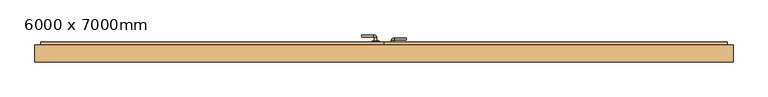
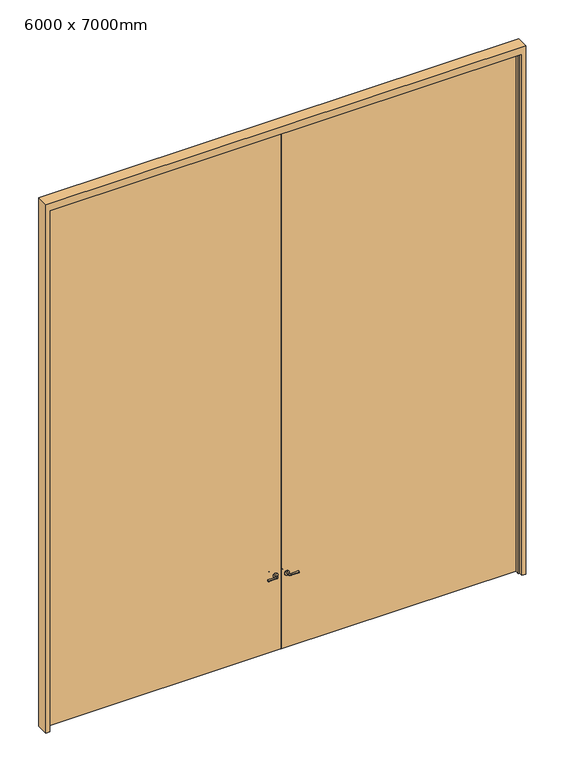
"""IFC4 building model written with IfcOpenShell, lengths in millimetres: door geometry, M_Puerta-De_paso-Doble-Paneles_planos : 6000 x 7000mm."""

from ifc_helpers import new_model, si_unit, point, frame, frame_2d, origin, origin_with_axes, place, context, project, spatial, polyline, circle_curve, ellipse_curve, trimmed, segment, composite_curve, outline, extrude, faceted_brep, source, transform, mapped, element, save
from ifc_brep_helpers import plane_surface, cylinder_surface, revolved_surface, advanced_brep


def door_6000_x_7000mm_428d85bf(model_context):
    return source(origin(), model_context, "Body", "SolidModel", [
        advanced_brep(
        [(-65.009375, 3.35, 1016.0), (-85.009375, 3.35, 1016.0), (-65.009375, -26.65, 1016.0), (-85.009375, -26.65, 1016.0), (-90.009375, -31.65, 1016.0), (-90.009375, -51.65, 1016.0), (-195.009375, -51.65, 1016.0), (-195.009375, -31.65, 1016.0)],
        [
            (0, 1, circle_curve(frame((-75.009375, 3.35, 1016.0), z_axis=(0.0, 1.0, 0.0), x_axis=(-1.0, 0.0, 0.0)), 10.0)),
            (1, 0, circle_curve(frame((-75.009375, 3.35, 1016.0), z_axis=(0.0, 1.0, 0.0), x_axis=(-1.0, 0.0, 0.0)), 10.0)),
            (0, 2),
            (2, 3, circle_curve(frame((-75.009375, -26.65, 1016.0), z_axis=(0.0, 1.0, 0.0), x_axis=(-1.0, 0.0, 0.0)), 10.0)),
            (3, 1),
            (3, 2, circle_curve(frame((-75.009375, -26.65, 1016.0), z_axis=(0.0, 1.0, 0.0), x_axis=(-1.0, 0.0, 0.0)), 10.0)),
            (4, 3, circle_curve(frame((-90.009375, -26.65, 1016.0), z_axis=(0.0, 0.0, 1.0), x_axis=(1.0, 0.0, 0.0)), 5.0)),
            (2, 5, circle_curve(frame((-90.009375, -26.65, 1016.0), z_axis=(0.0, 0.0, -1.0), x_axis=(1.0, 0.0, 0.0)), 25.0)),
            (5, 4, circle_curve(frame((-90.009375, -41.65, 1016.0), z_axis=(1.0, 0.0, 0.0), x_axis=(0.0, 1.0, 0.0)), 10.0)),
            (4, 5, circle_curve(frame((-90.009375, -41.65, 1016.0), z_axis=(1.0, 0.0, 0.0), x_axis=(0.0, 1.0, 0.0)), 10.0)),
            (6, 7, circle_curve(frame((-195.009375, -41.65, 1016.0), z_axis=(-1.0, 0.0, 0.0), x_axis=(0.0, 1.0, 0.0)), 10.0)),
            (7, 6, circle_curve(frame((-195.009375, -41.65, 1016.0), z_axis=(-1.0, 0.0, 0.0), x_axis=(0.0, 1.0, 0.0)), 10.0)),
            (5, 6),
            (7, 4),
        ],
        [
            plane_surface(frame((-75.009375, 3.35, 1016.0), z_axis=(0.0, 1.0, 0.0), x_axis=(0.0, 0.0, 1.0))),
            cylinder_surface(frame((-75.009375, 3.35, 1016.0), z_axis=(0.0, 1.0, 0.0), x_axis=(-1.0, 0.0, 0.0)), 10.0),
            revolved_surface(trimmed(ellipse_curve(frame((-75.009375, -26.65, 1016.0), z_axis=(0.0, 1.0, 0.0), x_axis=(-1.0, 0.0, 0.0)), 10.0, 10.0), [point((-65.009375, -26.65, 1016.0))], [point((-85.009375, -26.65, 1016.0))], True, "CARTESIAN"), (-90.009375, -26.65, 1016.0), (0.0, 0.0, -1.0)),
            revolved_surface(trimmed(ellipse_curve(frame((-75.009375, -26.65, 1016.0), z_axis=(0.0, 1.0, 0.0), x_axis=(-1.0, 0.0, 0.0)), 10.0, 10.0), [point((-85.009375, -26.65, 1016.0))], [point((-65.009375, -26.65, 1016.0))], True, "CARTESIAN"), (-90.009375, -26.65, 1016.0), (0.0, 0.0, -1.0)),
            plane_surface(frame((-195.009375, -41.65, 1016.0), z_axis=(-1.0, 0.0, 0.0), x_axis=(0.0, 0.0, 1.0))),
            cylinder_surface(frame((-90.009375, -41.65, 1016.0), z_axis=(1.0, 0.0, 0.0), x_axis=(0.0, 1.0, 0.0)), 10.0),
        ],
        [
            (0, [[1, 2]]),
            (1, [[-1, 3, 4, 5]]),
            (1, [[-2, -5, 6, -3]]),
            (2, [[7, -4, 8, 9]]),
            (3, [[-8, -6, -7, 10]]),
            (4, [[11, 12]]),
            (5, [[-9, 13, -12, 14]]),
            (5, [[-10, -14, -11, -13]]),
        ],
    ),
        extrude(outline(composite_curve([segment(trimmed(circle_curve(frame_2d((1016.0, -72.509375)), 30.0), [point((1016.0, -42.509375))], [point((1016.0, -102.509375))], False, "CARTESIAN"), True, "CONTINUOUS"), segment(trimmed(circle_curve(frame_2d((1016.0, -72.509375)), 30.0), [point((1016.0, -102.509375))], [point((1016.0, -42.509375))], False, "CARTESIAN"), True, "CONTINUOUS")], self_intersect=False)), frame((0.0, 3.35, 0.0), z_axis=(0.0, 1.0, 0.0), x_axis=(0.0, 0.0, 1.0)), (0.0, 0.0, 1.0), 8.0),
        advanced_brep(
        [(-65.009375, 90.95, 1000.0), (-85.009375, 90.95, 1000.0), (-85.009375, 120.95, 1000.0), (-65.009375, 120.95, 1000.0), (-90.009375, 125.95, 1000.0), (-90.009375, 145.95, 1000.0), (-195.009375, 145.95, 1000.0), (-195.009375, 125.95, 1000.0)],
        [
            (0, 1, circle_curve(frame((-75.009375, 90.95, 1000.0), z_axis=(0.0, -1.0, 0.0), x_axis=(-1.0, 0.0, 0.0)), 10.0)),
            (1, 0, circle_curve(frame((-75.009375, 90.95, 1000.0), z_axis=(0.0, -1.0, 0.0), x_axis=(-1.0, 0.0, 0.0)), 10.0)),
            (1, 2),
            (2, 3, circle_curve(frame((-75.009375, 120.95, 1000.0), z_axis=(0.0, -1.0, 0.0), x_axis=(-1.0, 0.0, 0.0)), 10.0)),
            (3, 0),
            (3, 2, circle_curve(frame((-75.009375, 120.95, 1000.0), z_axis=(0.0, -1.0, 0.0), x_axis=(-1.0, 0.0, 0.0)), 10.0)),
            (4, 5, circle_curve(frame((-90.009375, 135.95, 1000.0), z_axis=(1.0, 0.0, 0.0), x_axis=(0.0, -1.0, 0.0)), 10.0)),
            (5, 3, circle_curve(frame((-90.009375, 120.95, 1000.0), z_axis=(0.0, 0.0, -1.0), x_axis=(1.0, 0.0, 0.0)), 25.0)),
            (2, 4, circle_curve(frame((-90.009375, 120.95, 1000.0), z_axis=(0.0, 0.0, 1.0), x_axis=(1.0, 0.0, 0.0)), 5.0)),
            (5, 4, circle_curve(frame((-90.009375, 135.95, 1000.0), z_axis=(1.0, 0.0, 0.0), x_axis=(0.0, -1.0, 0.0)), 10.0)),
            (6, 7, circle_curve(frame((-195.009375, 135.95, 1000.0), z_axis=(-1.0, 0.0, 0.0), x_axis=(0.0, -1.0, 0.0)), 10.0)),
            (7, 6, circle_curve(frame((-195.009375, 135.95, 1000.0), z_axis=(-1.0, 0.0, 0.0), x_axis=(0.0, -1.0, 0.0)), 10.0)),
            (4, 7),
            (6, 5),
        ],
        [
            plane_surface(frame((-75.009375, 90.95, 1000.0), z_axis=(0.0, -1.0, 0.0), x_axis=(0.0, 0.0, 1.0))),
            cylinder_surface(frame((-75.009375, 90.95, 1000.0), z_axis=(0.0, -1.0, 0.0), x_axis=(-1.0, 0.0, 0.0)), 10.0),
            revolved_surface(trimmed(ellipse_curve(frame((-75.009375, 120.95, 1000.0), z_axis=(0.0, 1.0, 0.0), x_axis=(-1.0, 0.0, 0.0)), 10.0, 10.0), [point((-65.009375, 120.95, 1000.0))], [point((-85.009375, 120.95, 1000.0))], True, "CARTESIAN"), (-90.009375, 120.95, 1000.0), (0.0, 0.0, -1.0)),
            revolved_surface(trimmed(ellipse_curve(frame((-75.009375, 120.95, 1000.0), z_axis=(0.0, 1.0, 0.0), x_axis=(-1.0, 0.0, 0.0)), 10.0, 10.0), [point((-85.009375, 120.95, 1000.0))], [point((-65.009375, 120.95, 1000.0))], True, "CARTESIAN"), (-90.009375, 120.95, 1000.0), (0.0, 0.0, -1.0)),
            plane_surface(frame((-195.009375, 135.95, 1000.0), z_axis=(-1.0, 0.0, 0.0), x_axis=(0.0, 0.0, 1.0))),
            cylinder_surface(frame((-90.009375, 135.95, 1000.0), z_axis=(1.0, 0.0, 0.0), x_axis=(0.0, -1.0, 0.0)), 10.0),
        ],
        [
            (0, [[1, 2]]),
            (1, [[3, 4, 5, -2]]),
            (1, [[-5, 6, -3, -1]]),
            (2, [[7, 8, -4, 9]]),
            (3, [[10, -9, -6, -8]]),
            (4, [[11, 12]]),
            (5, [[13, -11, 14, -7]]),
            (5, [[-14, -12, -13, -10]]),
        ],
    ),
        extrude(outline(composite_curve([segment(trimmed(circle_curve(frame_2d((1000.0, -72.509375)), 30.0), [point((1000.0, -42.509375))], [point((1000.0, -102.509375))], False, "CARTESIAN"), True, "CONTINUOUS"), segment(trimmed(circle_curve(frame_2d((1000.0, -72.509375)), 30.0), [point((1000.0, -102.509375))], [point((1000.0, -42.509375))], False, "CARTESIAN"), True, "CONTINUOUS")], self_intersect=False)), frame((0.0, 82.95, 0.0), z_axis=(0.0, 1.0, 0.0), x_axis=(0.0, 0.0, 1.0)), (0.0, 0.0, 1.0), 8.0),
        advanced_brep(
        [(65.009375, 3.35, 1000.0), (85.009375, 3.35, 1000.0), (85.009375, -26.65, 1000.0), (65.009375, -26.65, 1000.0), (90.009375, -31.65, 1000.0), (90.009375, -51.65, 1000.0), (195.009375, -51.65, 1000.0), (195.009375, -31.65, 1000.0)],
        [
            (0, 1, circle_curve(frame((75.009375, 3.35, 1000.0), z_axis=(0.0, 1.0, 0.0), x_axis=(1.0, 0.0, 0.0)), 10.0)),
            (1, 0, circle_curve(frame((75.009375, 3.35, 1000.0), z_axis=(0.0, 1.0, 0.0), x_axis=(1.0, 0.0, 0.0)), 10.0)),
            (1, 2),
            (2, 3, circle_curve(frame((75.009375, -26.65, 1000.0), z_axis=(0.0, 1.0, 0.0), x_axis=(1.0, 0.0, 0.0)), 10.0)),
            (3, 0),
            (3, 2, circle_curve(frame((75.009375, -26.65, 1000.0), z_axis=(0.0, 1.0, 0.0), x_axis=(1.0, 0.0, 0.0)), 10.0)),
            (4, 5, circle_curve(frame((90.009375, -41.65, 1000.0), z_axis=(-1.0, 0.0, 0.0), x_axis=(0.0, 1.0, 0.0)), 10.0)),
            (5, 3, circle_curve(frame((90.009375, -26.65, 1000.0), z_axis=(0.0, 0.0, -1.0), x_axis=(-1.0, 0.0, 0.0)), 25.0)),
            (2, 4, circle_curve(frame((90.009375, -26.65, 1000.0), z_axis=(0.0, 0.0, 1.0), x_axis=(-1.0, 0.0, 0.0)), 5.0)),
            (5, 4, circle_curve(frame((90.009375, -41.65, 1000.0), z_axis=(-1.0, 0.0, 0.0), x_axis=(0.0, 1.0, 0.0)), 10.0)),
            (6, 7, circle_curve(frame((195.009375, -41.65, 1000.0), z_axis=(1.0, 0.0, 0.0), x_axis=(0.0, 1.0, 0.0)), 10.0)),
            (7, 6, circle_curve(frame((195.009375, -41.65, 1000.0), z_axis=(1.0, 0.0, 0.0), x_axis=(0.0, 1.0, 0.0)), 10.0)),
            (4, 7),
            (6, 5),
        ],
        [
            plane_surface(frame((75.009375, 3.35, 1000.0), z_axis=(0.0, 1.0, 0.0), x_axis=(0.0, 0.0, 1.0))),
            cylinder_surface(frame((75.009375, 3.35, 1000.0), z_axis=(0.0, 1.0, 0.0), x_axis=(1.0, 0.0, 0.0)), 10.0),
            revolved_surface(trimmed(ellipse_curve(frame((75.009375, -26.65, 1000.0), z_axis=(0.0, -1.0, 0.0), x_axis=(1.0, 0.0, 0.0)), 10.0, 10.0), [point((65.009375, -26.65, 1000.0))], [point((85.009375, -26.65, 1000.0))], True, "CARTESIAN"), (90.009375, -26.65, 1000.0), (0.0, 0.0, -1.0)),
            revolved_surface(trimmed(ellipse_curve(frame((75.009375, -26.65, 1000.0), z_axis=(0.0, -1.0, 0.0), x_axis=(1.0, 0.0, 0.0)), 10.0, 10.0), [point((85.009375, -26.65, 1000.0))], [point((65.009375, -26.65, 1000.0))], True, "CARTESIAN"), (90.009375, -26.65, 1000.0), (0.0, 0.0, -1.0)),
            plane_surface(frame((195.009375, -41.65, 1000.0), z_axis=(1.0, 0.0, 0.0), x_axis=(0.0, 0.0, 1.0))),
            cylinder_surface(frame((90.009375, -41.65, 1000.0), z_axis=(-1.0, 0.0, 0.0), x_axis=(0.0, 1.0, 0.0)), 10.0),
        ],
        [
            (0, [[1, 2]]),
            (1, [[3, 4, 5, -2]]),
            (1, [[-5, 6, -3, -1]]),
            (2, [[7, 8, -4, 9]]),
            (3, [[10, -9, -6, -8]]),
            (4, [[11, 12]]),
            (5, [[13, -11, 14, -7]]),
            (5, [[-14, -12, -13, -10]]),
        ],
    ),
        extrude(outline(composite_curve([segment(trimmed(circle_curve(frame_2d((1000.0, 72.509375)), 30.0), [point((1000.0, 42.509375))], [point((1000.0, 102.509375))], False, "CARTESIAN"), True, "CONTINUOUS"), segment(trimmed(circle_curve(frame_2d((1000.0, 72.509375)), 30.0), [point((1000.0, 102.509375))], [point((1000.0, 42.509375))], False, "CARTESIAN"), True, "CONTINUOUS")], self_intersect=False)), frame((0.0, 3.35, 0.0), z_axis=(0.0, 1.0, 0.0), x_axis=(0.0, 0.0, 1.0)), (0.0, 0.0, 1.0), 8.0),
        advanced_brep(
        [(65.009375, 64.35, 1000.0), (85.009375, 64.35, 1000.0), (65.009375, 94.35, 1000.0), (85.009375, 94.35, 1000.0), (90.009375, 99.35, 1000.0), (90.009375, 119.35, 1000.0), (195.009375, 119.35, 1000.0), (195.009375, 99.35, 1000.0)],
        [
            (0, 1, circle_curve(frame((75.009375, 64.35, 1000.0), z_axis=(0.0, -1.0, 0.0), x_axis=(1.0, 0.0, 0.0)), 10.0)),
            (1, 0, circle_curve(frame((75.009375, 64.35, 1000.0), z_axis=(0.0, -1.0, 0.0), x_axis=(1.0, 0.0, 0.0)), 10.0)),
            (0, 2),
            (2, 3, circle_curve(frame((75.009375, 94.35, 1000.0), z_axis=(0.0, -1.0, 0.0), x_axis=(1.0, 0.0, 0.0)), 10.0)),
            (3, 1),
            (3, 2, circle_curve(frame((75.009375, 94.35, 1000.0), z_axis=(0.0, -1.0, 0.0), x_axis=(1.0, 0.0, 0.0)), 10.0)),
            (4, 3, circle_curve(frame((90.009375, 94.35, 1000.0), z_axis=(0.0, 0.0, 1.0), x_axis=(-1.0, 0.0, 0.0)), 5.0)),
            (2, 5, circle_curve(frame((90.009375, 94.35, 1000.0), z_axis=(0.0, 0.0, -1.0), x_axis=(-1.0, 0.0, 0.0)), 25.0)),
            (5, 4, circle_curve(frame((90.009375, 109.35, 1000.0), z_axis=(-1.0, 0.0, 0.0), x_axis=(0.0, -1.0, 0.0)), 10.0)),
            (4, 5, circle_curve(frame((90.009375, 109.35, 1000.0), z_axis=(-1.0, 0.0, 0.0), x_axis=(0.0, -1.0, 0.0)), 10.0)),
            (6, 7, circle_curve(frame((195.009375, 109.35, 1000.0), z_axis=(1.0, 0.0, 0.0), x_axis=(0.0, -1.0, 0.0)), 10.0)),
            (7, 6, circle_curve(frame((195.009375, 109.35, 1000.0), z_axis=(1.0, 0.0, 0.0), x_axis=(0.0, -1.0, 0.0)), 10.0)),
            (5, 6),
            (7, 4),
        ],
        [
            plane_surface(frame((75.009375, 64.35, 1000.0), z_axis=(0.0, -1.0, 0.0), x_axis=(0.0, 0.0, 1.0))),
            cylinder_surface(frame((75.009375, 64.35, 1000.0), z_axis=(0.0, -1.0, 0.0), x_axis=(1.0, 0.0, 0.0)), 10.0),
            revolved_surface(trimmed(ellipse_curve(frame((75.009375, 94.35, 1000.0), z_axis=(0.0, -1.0, 0.0), x_axis=(1.0, 0.0, 0.0)), 10.0, 10.0), [point((65.009375, 94.35, 1000.0))], [point((85.009375, 94.35, 1000.0))], True, "CARTESIAN"), (90.009375, 94.35, 1000.0), (0.0, 0.0, -1.0)),
            revolved_surface(trimmed(ellipse_curve(frame((75.009375, 94.35, 1000.0), z_axis=(0.0, -1.0, 0.0), x_axis=(1.0, 0.0, 0.0)), 10.0, 10.0), [point((85.009375, 94.35, 1000.0))], [point((65.009375, 94.35, 1000.0))], True, "CARTESIAN"), (90.009375, 94.35, 1000.0), (0.0, 0.0, -1.0)),
            plane_surface(frame((195.009375, 109.35, 1000.0), z_axis=(1.0, 0.0, 0.0), x_axis=(0.0, 0.0, 1.0))),
            cylinder_surface(frame((90.009375, 109.35, 1000.0), z_axis=(-1.0, 0.0, 0.0), x_axis=(0.0, -1.0, 0.0)), 10.0),
        ],
        [
            (0, [[1, 2]]),
            (1, [[-1, 3, 4, 5]]),
            (1, [[-2, -5, 6, -3]]),
            (2, [[7, -4, 8, 9]]),
            (3, [[-8, -6, -7, 10]]),
            (4, [[11, 12]]),
            (5, [[-9, 13, -12, 14]]),
            (5, [[-10, -14, -11, -13]]),
        ],
    ),
        extrude(outline(composite_curve([segment(trimmed(circle_curve(frame_2d((1000.0, 72.509375)), 30.0), [point((1000.0, 42.509375))], [point((1000.0, 102.509375))], False, "CARTESIAN"), True, "CONTINUOUS"), segment(trimmed(circle_curve(frame_2d((1000.0, 72.509375)), 30.0), [point((1000.0, 102.509375))], [point((1000.0, 42.509375))], False, "CARTESIAN"), True, "CONTINUOUS")], self_intersect=False)), frame((0.0, 56.35, 0.0), z_axis=(0.0, 1.0, 0.0), x_axis=(0.0, 0.0, 1.0)), (0.0, 0.0, 1.0), 8.0),
        extrude(outline(polyline([(3000.0, 11.35), (1.5875, 11.35), (1.5875, 82.95), (3000.0, 82.95), (3000.0, 11.35)])), origin_with_axes(), (0.0, 0.0, 1.0), 7000.0),
        extrude(outline(polyline([(-1.5875, 11.35), (-3000.0, 11.35), (-3000.0, 82.95), (-1.5875, 82.95), (-1.5875, 11.35)])), origin_with_axes(), (0.0, 0.0, 1.0), 7000.0),
        faceted_brep([(3000.0, 6.5875, 0.0), (3000.0, 56.35, 0.0), (3050.0, 56.35, 0.0), (3050.0, -93.65, 0.0), (3000.0, -93.65, 0.0), (3000.0, -44.4375, 0.0), (2984.125, -44.4375, 0.0), (2984.125, 6.5875, 0.0), (3000.0, 6.5875, 7000.0), (3000.0, 56.35, 7000.0), (-3000.0, 56.35, 7000.0), (-3000.0, 56.35, 0.0), (-3050.0, 56.35, 0.0), (-3050.0, 56.35, 7100.0), (3050.0, 56.35, 7100.0), (3050.0, -93.65, 7100.0), (-3050.0, -93.65, 7100.0), (-3050.0, -93.65, 0.0), (-3000.0, -93.65, 0.0), (-3000.0, -93.65, 7000.0), (3000.0, -93.65, 7000.0), (3000.0, -44.4375, 7000.0), (-3000.0, -44.4375, 7000.0), (-3000.0, -44.4375, 0.0), (-2984.125, -44.4375, 0.0), (-2984.125, -44.4375, 6984.125), (2984.125, -44.4375, 6984.125), (2984.125, 6.5875, 6984.125), (-2984.125, 6.5875, 6984.125), (-2984.125, 6.5875, 0.0), (-3000.0, 6.5875, 0.0), (-3000.0, 6.5875, 7000.0)], [[[0, 1, 2, 3, 4, 5, 6, 7]], [[1, 0, 8, 9]], [[2, 1, 9, 10, 11, 12, 13, 14]], [[3, 2, 14, 15]], [[4, 3, 15, 16, 17, 18, 19, 20]], [[5, 4, 20, 21]], [[6, 5, 21, 22, 23, 24, 25, 26]], [[7, 6, 26, 27]], [[0, 7, 27, 28, 29, 30, 31, 8]], [[9, 8, 31, 10]], [[20, 19, 22, 21]], [[26, 25, 28, 27]], [[12, 11, 30, 29, 24, 23, 18, 17]], [[11, 10, 31, 30]], [[13, 12, 17, 16]], [[19, 18, 23, 22]], [[25, 24, 29, 28]], [[15, 14, 13, 16]]]),
    ])


if __name__ == "__main__":
    model = new_model("IFC4")
    model_context = context("Model", 3, world=origin())
    ifc_project = project(units=[si_unit("LENGTHUNIT", "METRE", prefix="MILLI")], contexts=[model_context])
    site = spatial("IfcSite", under=ifc_project)
    building = spatial("IfcBuilding", under=site)
    placement = place(None, origin())
    door_6000_x_7000mm_shape = door_6000_x_7000mm_428d85bf(model_context)
    element("IfcDoor", 1, ObjectType="M_Puerta-De_paso-Doble-Paneles_planos : 6000 x 7000mm", at=placement, inside=building, context=model_context, shape_type="MappedRepresentation", body=[
        mapped(door_6000_x_7000mm_shape, transform((0.0, 0.0, 0.0), x_axis=(1.0, 0.0, 0.0), y_axis=(0.0, 1.0, 0.0), z_axis=(0.0, 0.0, 1.0))),
    ])
    save(model, "model.ifc")

# Revit data of these elements
# Type "M_Puerta-De_paso-Doble-Paneles_planos : 6000 x 7000mm"
#   Type Mark = "48"
#   Analytic Construction = "Metal"
#   Thickness = 0.045 m
#   Thermal Resistance (R) = 0.270118 (m²·K)/W
#   Ángulo de batiente [instance default] = 90.00°
#   Altura del pasador = 1.00 m
#   Anchura de panel simple = 3.00 m
#   Rough Width [instance default] = 6.10 m
#   Rough Height [instance default] = 7.10 m
#   MFAltura de hueco [instance default] = 0.10 m
#   MFAnchura de hueco [instance default] = 0.10 m
#   Cálculo de la incrustación [instance default] = 0.105 m
#   Incrustación de albañilería [instance default] = 0.025 m
#   Height = 7.00 m
#   Width = 6.00 m
#   Heat Transfer Coefficient (U) = 3.70223 W/(m²·K)
#   Profundidad del marco del albañilería = 0.15 m
#   Marco del albañilería [instance default] = yes
#   Function = 1
#   Marco de muro seco [instance default] = no
#   Material de panel = Puerta de metal - Pinto
#   Material de estructura = Metal - Pintado - Gris
#   Material de tirador = Aluminio 1
#   Visual Light Transmittance = 0
#   Solar Heat Gain Coefficient = 0
#   Wall Closure = (empty or 0)
# Element 1 (IfcDoor, "M_Puerta-De_paso-Doble-Paneles_planos : 6000 x 7000mm")
#   Materials on its faces: "Aluminio 1", "Metal - Pintado - Gris", "Puerta de metal - Pinto"
# Materials
#   "Puerta de metal - Pinto": class "Pintura", colour RGB 164 133 98, transparency 0
#   "Metal - Pintado - Gris": class "Pintura", colour RGB 104 104 104, transparency 0
#   "Aluminio 1": class "Metal", colour RGB 244 245 246, transparency 0, Description = "Aluminio 6061", Cost = 0
